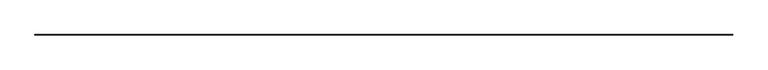
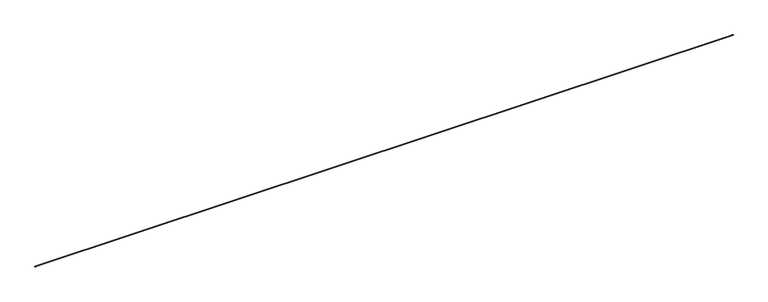
"""IFC4 building model written with IfcOpenShell, lengths in millimetres: proxy geometry, Generic Models 7:Generic Models 1:1:Generic Models 1:1 : Generic Models 7:Generic Models 1:337419:3 : Generic Models 7:Generic Models 1:1:Generic Models 1:1 : Generic Models 7:Generic Models 1:337419:306201."""

import ifcopenshell
import ifcopenshell.guid

model = None  # the IFC model being written
_history = None  # IfcOwnerHistory: only IFC2X3 demands one
_inside = {}  # id of a spatial element -> (the spatial element, [elements in it])
_under = {}  # id of a project, library or spatial element -> (it, [spatial elements below it])
_declared = {}  # id of a project -> (the project, [libraries it declares])
_typed = {}  # id of a type object -> (the type object, [elements of that type])
_made_of = {}  # id of a material, layer set ... -> (it, [elements and type objects made of it])


def new_model(schema):
    """Start an empty IFC model of exactly this schema.

    Asked for "IFC4X3", IfcOpenShell would pick the latest addendum, in which some entities
    have other attributes; the version numbers below select the first issue.
    IFC2X3 requires an IfcOwnerHistory on every rooted entity: one is made here for all.
    """
    global model, _history
    if schema == "IFC4X3":
        model = ifcopenshell.file(schema_version=(4, 3, 0, 0))
    else:
        model = ifcopenshell.file(schema=schema)
    _inside.clear()
    _under.clear()
    _declared.clear()
    _typed.clear()
    _made_of.clear()
    _history = None
    if model.schema == "IFC2X3":
        org = make("IfcOrganization", Name="unknown")
        user = make(
            "IfcPersonAndOrganization",
            ThePerson=make("IfcPerson", FamilyName="unknown"),
            TheOrganization=org,
        )
        app = make(
            "IfcApplication",
            ApplicationDeveloper=org,
            Version="unknown",
            ApplicationFullName="unknown",
            ApplicationIdentifier="unknown",
        )
        _history = make(
            "IfcOwnerHistory",
            OwningUser=user,
            OwningApplication=app,
            ChangeAction="ADDED",
            CreationDate=0,
        )
    return model


def make(cls, **values):
    """One entity of the class cls with the attributes given. An attribute that is None is left unset."""
    return model.create_entity(
        cls, **{name: value for name, value in values.items() if value is not None}
    )


def rooted(cls, **values):
    """An entity with a GlobalId (a new one), such as an element, a storey or a relation."""
    return make(cls, GlobalId=ifcopenshell.guid.new(), OwnerHistory=_history, **values)


def si_unit(unit_type, name, prefix=None):
    """IfcSIUnit, for example si_unit("LENGTHUNIT", "METRE", prefix="MILLI")."""
    return make("IfcSIUnit", UnitType=unit_type, Prefix=prefix, Name=name)


def assignment(units):
    """IfcUnitAssignment: the units of a project."""
    return None if units is None else make("IfcUnitAssignment", Units=units)


def point(xyz):
    """IfcCartesianPoint."""
    return None if xyz is None else make("IfcCartesianPoint", Coordinates=xyz)


def direction(xyz):
    """IfcDirection."""
    return None if xyz is None else make("IfcDirection", DirectionRatios=xyz)


def frame(location, z_axis=None, x_axis=None):
    """IfcAxis2Placement3D, a coordinate frame: its origin and axes. An axis left out is left unset."""
    return make(
        "IfcAxis2Placement3D",
        Location=point(location),
        Axis=direction(z_axis),
        RefDirection=direction(x_axis),
    )


def origin():
    """The frame at (0, 0, 0) with its axes left unset."""
    return frame((0.0, 0.0, 0.0))


def place(relative_to, where):
    """IfcLocalPlacement: puts the frame where relative to a parent placement (None: the world)."""
    return make(
        "IfcLocalPlacement", PlacementRelTo=relative_to, RelativePlacement=where
    )


def context(
    kind, dimensions, precision=None, world=None, true_north=None, identifier=None
):
    """IfcGeometricRepresentationContext, for example the 3D "Model" context."""
    return make(
        "IfcGeometricRepresentationContext",
        ContextIdentifier=identifier,
        ContextType=kind,
        CoordinateSpaceDimension=dimensions,
        Precision=precision,
        WorldCoordinateSystem=world,
        TrueNorth=true_north,
    )


def project(units=None, contexts=None):
    """IfcProject with its units and contexts."""
    return rooted(
        "IfcProject",
        Name="project",
        RepresentationContexts=contexts,
        UnitsInContext=assignment(units),
    )


def spatial(cls, under=None, at=None, **own):
    """A site, building, storey or space (cls), placed at a placement, below another one or the project."""
    s = rooted(cls, ObjectPlacement=at, **own)
    if under is not None:
        _under.setdefault(under.id(), (under, []))[1].append(s)
    return s


def polyline(points):
    """IfcPolyline through the points."""
    return make("IfcPolyline", Points=[point(p) for p in points])


def outline(outer, holes=None, kind="AREA"):
    """IfcArbitraryClosedProfileDef: a profile drawn as a closed curve; with holes, ...WithVoids."""
    if holes is None:
        return make("IfcArbitraryClosedProfileDef", ProfileType=kind, OuterCurve=outer)
    return make(
        "IfcArbitraryProfileDefWithVoids",
        ProfileType=kind,
        OuterCurve=outer,
        InnerCurves=holes,
    )


def extrude(swept, where, along, depth):
    """IfcExtrudedAreaSolid: the profile swept, set in the frame where, extruded along a direction by depth."""
    return make(
        "IfcExtrudedAreaSolid",
        SweptArea=swept,
        Position=where,
        ExtrudedDirection=direction(along),
        Depth=depth,
    )


def shape(context_of_items, identifier, shape_type, items):
    """IfcShapeRepresentation: the items that make up one representation, for example the "Body"."""
    return make(
        "IfcShapeRepresentation",
        ContextOfItems=context_of_items,
        RepresentationIdentifier=identifier,
        RepresentationType=shape_type,
        Items=items,
    )


def source(mapping_origin, context_of_items, identifier, shape_type, items):
    """IfcRepresentationMap: a shape defined once, which mapped items show again and again."""
    return make(
        "IfcRepresentationMap",
        MappingOrigin=mapping_origin,
        MappedRepresentation=shape(context_of_items, identifier, shape_type, items),
    )


def transform(
    local_origin,
    x_axis=None,
    y_axis=None,
    z_axis=None,
    scale=None,
    scale2=None,
    scale3=None,
    uniform=True,
):
    """IfcCartesianTransformationOperator3D, or its non-uniform kind. x_axis, y_axis, z_axis: its Axis1, 2, 3."""
    if uniform:
        return make(
            "IfcCartesianTransformationOperator3D",
            Axis1=direction(x_axis),
            Axis2=direction(y_axis),
            LocalOrigin=point(local_origin),
            Scale=scale,
            Axis3=direction(z_axis),
        )
    return make(
        "IfcCartesianTransformationOperator3DnonUniform",
        Axis1=direction(x_axis),
        Axis2=direction(y_axis),
        LocalOrigin=point(local_origin),
        Scale=scale,
        Axis3=direction(z_axis),
        Scale2=scale2,
        Scale3=scale3,
    )


def mapped(mapping_source, mapping_target):
    """IfcMappedItem: shows the shape of a source again, moved by a transform."""
    return make(
        "IfcMappedItem", MappingSource=mapping_source, MappingTarget=mapping_target
    )


def made_of(thing, what):
    """Note that an element or type object is made of a material, layer set ...; save() writes the relation."""
    if what is not None:
        _made_of.setdefault(what.id(), (what, []))[1].append(thing)
    return thing


def element(
    cls,
    number,
    at=None,
    inside=None,
    cuts=None,
    type_object=None,
    material=None,
    context=None,
    identifier="Body",
    shape_type=None,
    held_by="IfcProductDefinitionShape",
    body=None,
    shapes=None,
    **own,
):
    """One element of the class cls, such as IfcWall. Its Tag is "e" and its number.

    at: its placement. inside: the storey or other place that contains it. cuts: it is an
    opening in that element (IfcRelVoidsElement). A single representation is given by context,
    identifier, shape_type and body (its items); several are given by shapes. held_by: the class
    of the entity that holds the representations. save() writes the other relations.
    """
    e = rooted(cls, Tag="e%d" % number, ObjectPlacement=at, **own)
    if body is not None:
        shapes = [shape(context, identifier, shape_type, body)]
    if shapes is not None:
        e.Representation = make(held_by, Representations=shapes)
    if inside is not None:
        _inside.setdefault(inside.id(), (inside, []))[1].append(e)
    if cuts is not None:
        rooted(
            "IfcRelVoidsElement", RelatingBuildingElement=cuts, RelatedOpeningElement=e
        )
    if type_object is not None:
        _typed.setdefault(type_object.id(), (type_object, []))[1].append(e)
    return made_of(e, material)


def aggregate(whole, parts):
    """IfcRelAggregates: a whole, such as a stair, and the parts it consists of."""
    return rooted("IfcRelAggregates", RelatingObject=whole, RelatedObjects=parts)


def save(model, path):
    """Write the relations noted so far, then the file.

    IfcRelAggregates (storeys below a building ...), IfcRelContainedInSpatialStructure (elements
    in a storey), IfcRelDefinesByType, IfcRelAssociatesMaterial and IfcRelDeclares: one each for
    every whole, place, type object, material and project.
    """
    for whole, parts in _under.values():
        aggregate(whole, parts)
    for where, things in _inside.values():
        rooted(
            "IfcRelContainedInSpatialStructure",
            RelatedElements=things,
            RelatingStructure=where,
        )
    for kind, things in _typed.values():
        rooted("IfcRelDefinesByType", RelatedObjects=things, RelatingType=kind)
    for what, things in _made_of.values():
        rooted("IfcRelAssociatesMaterial", RelatedObjects=things, RelatingMaterial=what)
    for by, libraries in _declared.values():
        rooted("IfcRelDeclares", RelatingContext=by, RelatedDefinitions=libraries)
    model.write(path)


def generic_models_0c188b81(model_context):
    return source(origin(), model_context, "Body", "SweptSolid", [
        extrude(outline(polyline([(-578873.6913841, -11.7361843), (-578874.4640193, -10.0156223), (-578876.6309901, -7.396472), (-578879.3314857, -6.195765), (-578882.1430382, -6.6013407), (-578884.6258064, -8.5497508), (-578886.3913841, -11.7361843), (-578886.3913841, 0.0), (-578884.4598576, -0.7548172), (-578880.0413841, -1.3821894), (-578875.6229105, -0.7548172), (-578873.6913841, 0.0), (-578873.6913841, -11.7361843)])), frame((557809.7867239, 0.0, 0.0), z_axis=(1.0, 0.0, 0.0), x_axis=(0.0, 1.0, 0.0)), (0.0, 0.0, 1.0), 38252.9096551),
        extrude(outline(polyline([(-578873.8505919, -18.5829513), (-578875.0767542, -22.4021798), (-578877.2862223, -25.0451679), (-578880.0413841, -25.9884394), (-578882.7965458, -25.0451679), (-578885.006014, -22.4021798), (-578886.2321763, -18.5829513), (-578886.3913841, -16.4634394), (-578886.2321763, -14.3439275), (-578885.006014, -10.524699), (-578882.7965458, -7.8817109), (-578880.0413841, -6.9384394), (-578877.2862223, -7.8817109), (-578875.0767542, -10.524699), (-578873.8505919, -14.3439275), (-578873.6913841, -16.4634394), (-578873.8505919, -18.5829513)])), frame((557809.7867239, 0.0, 0.0), z_axis=(1.0, 0.0, 0.0), x_axis=(0.0, 1.0, 0.0)), (0.0, 0.0, 1.0), 38252.9096551),
    ])


if __name__ == "__main__":
    model = new_model("IFC4")
    model_context = context("Model", 3, world=origin())
    ifc_project = project(units=[si_unit("LENGTHUNIT", "METRE", prefix="MILLI")], contexts=[model_context])
    site = spatial("IfcSite", under=ifc_project)
    building = spatial("IfcBuilding", under=site)
    placement = place(None, origin())
    generic_models_shape = generic_models_0c188b81(model_context)
    element("IfcBuildingElementProxy", 1, Name="Generic Models 7:Generic Models 1:1:Generic Models 1:1 : Generic Models 7:Generic Models 1:337419:3 : Generic Models 7:Generic Models 1:1:Generic Models 1:1 : Generic Models 7:Generic Models 1:337419:306201", ObjectType="Generic Models 7:Generic Models 1:1:Generic Models 1:1 : Generic Models 7:Generic Models 1:337419:3 : Generic Models 7:Generic Models 1:1:Generic Models 1:1 : Generic Models 7:Generic Models 1:337419:306201", at=placement, inside=building, context=model_context, shape_type="MappedRepresentation", body=[
        mapped(generic_models_shape, transform((0.0, 0.0, 0.0), x_axis=(1.0, 0.0, 0.0), y_axis=(0.0, 1.0, 0.0), z_axis=(0.0, 0.0, 1.0))),
    ])
    save(model, "model.ifc")

# Revit data of these elements
# Type "Generic Models 7:Generic Models 1:1:Generic Models 1:1 : Generic Models 7:Generic Models 1:337419:3 : Generic Models 7:Generic Models 1:1:Generic Models 1:1 : Generic Models 7:Generic Models 1:337419:306201"
#   NameOverride = "Generic Models 7:Generic Models 1:1:Generic Models 1:1 : Generic Models 7:Generic Models 1:337419:306201"
#   ObjectTypeOverride = "Generic Models 1:1 : Generic Models 7:Generic Models 1:337419"
#   Reference = "Generic Models 1"
#   Tag = "306201"
# Element 1 (IfcBuildingElementProxy, "Generic Models 7:Generic Models 1:1:Generic Models 1:1 : Generic Models 7:Generic Models 1:337419:3 : Generic Models 7:Generic Models 1:1:Generic Models 1:1 : Generic Models 7:Generic Models 1:337419:306201")
#   Materials on its faces: "SEMI-RIGID EPOXY SEALANT W/ BACKROD (REMOVE TEMP. JOINT FORM)"
# Materials
#   "SEMI-RIGID EPOXY SEALANT W/ BACKROD (REMOVE TEMP. JOINT FORM)": class "Unassigned", colour RGB 120 120 120, transparency 0, Cost = 0
